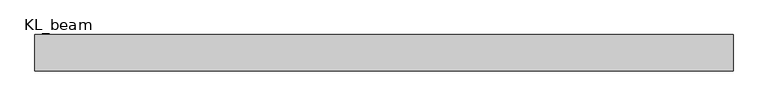
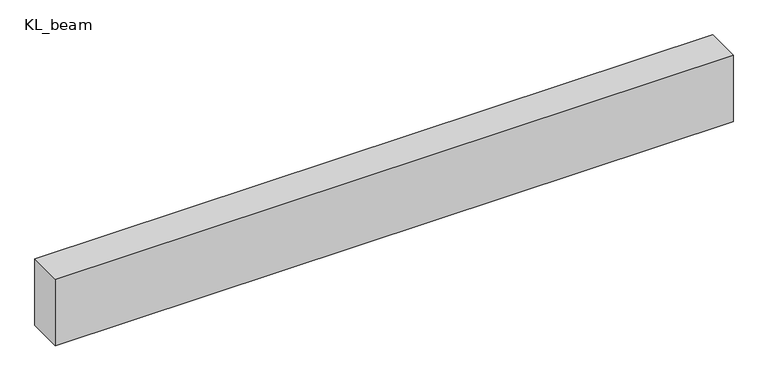
"""IFC4 building model written with IfcOpenShell, lengths in millimetres: beam geometry, 混凝土 - 矩形梁 : KL_beam."""

from ifc_helpers import new_model, si_unit, frame, origin, place, context, project, spatial, polyline, outline, extrude, source, transform, mapped, element, save


def kl_beam_eab3c69a(model_context):
    return source(origin(), model_context, "Body", "SweptSolid", [
        extrude(outline(polyline([(3851.0, 200.0), (3851.0, -200.0), (-3851.0, -200.0), (-3851.0, 200.0), (3851.0, 200.0)])), frame((0.0, 0.0, -400.0), z_axis=(0.0, 0.0, 1.0), x_axis=(1.0, 0.0, 0.0)), (0.0, 0.0, 1.0), 800.0),
    ])


if __name__ == "__main__":
    model = new_model("IFC4")
    model_context = context("Model", 3, world=origin())
    ifc_project = project(units=[si_unit("LENGTHUNIT", "METRE", prefix="MILLI")], contexts=[model_context])
    site = spatial("IfcSite", under=ifc_project)
    building = spatial("IfcBuilding", under=site)
    placement = place(None, origin())
    kl_beam_shape = kl_beam_eab3c69a(model_context)
    element("IfcBeam", 1, ObjectType="混凝土 - 矩形梁 : KL_beam", at=placement, inside=building, context=model_context, shape_type="MappedRepresentation", body=[
        mapped(kl_beam_shape, transform((0.0, 0.0, 0.0), x_axis=(1.0, 0.0, 0.0), y_axis=(0.0, 1.0, 0.0), z_axis=(0.0, 0.0, 1.0))),
    ])
    save(model, "model.ifc")

# Revit data of these elements
# Type "混凝土 - 矩形梁 : KL_beam"
#   Length [instance default] = 1524 mm
#   b = 400 mm
#   h = 800 mm
#   Structural Material [instance default] = 混凝土 - 现场浇注混凝土
#   Assembly Code = ""
# Element 1 (IfcBeam, "混凝土 - 矩形梁 : KL_beam")
#   Structural Material = none
# Materials
#   "混凝土 - 现场浇注混凝土": class "混凝土", colour RGB 192 192 192, transparency 0
